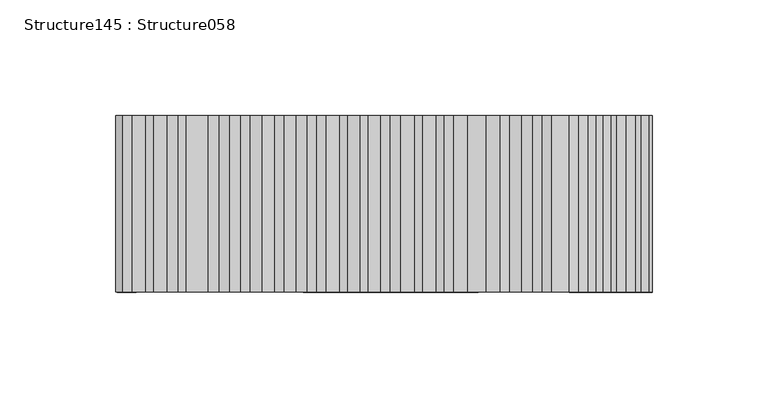
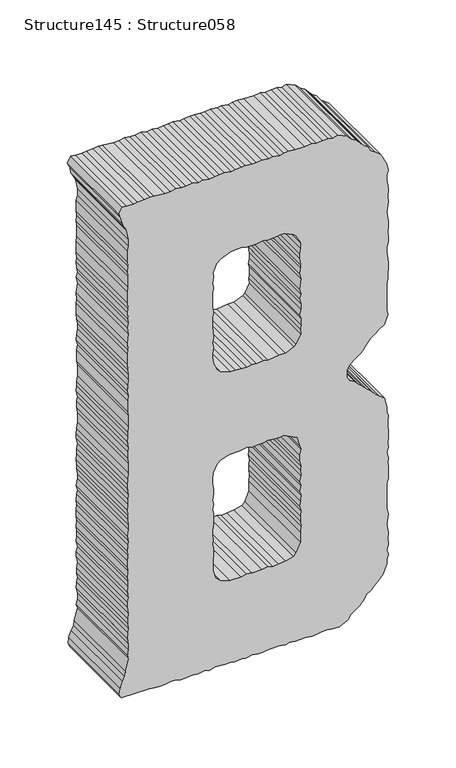
"""IFC4 building model written with IfcOpenShell, lengths in millimetres: proxy geometry, Structure145 : Structure058."""

from ifc_helpers import new_model, si_unit, frame, origin, place, context, project, spatial, polyline, outline, extrude, source, transform, mapped, element, save


def structure145_structure058_15f4931a(model_context):
    return source(origin(), model_context, "Body", "SweptSolid", [
        extrude(outline(polyline([(3581.5276686, -40098.3513957), (3585.0706354, -40095.4101556), (3593.2541183, -40091.9105132), (3597.3538828, -40091.9105132), (3601.4536473, -40090.7295243), (3606.1551384, -40091.9105132), (3610.838979, -40090.7295243), (3616.69739, -40091.331251), (3621.3732075, -40090.7295243), (3628.998288, -40091.9105132), (3638.3563415, -40090.7295243), (3644.2420307, -40091.9105132), (3666.5027089, -40091.9105132), (3670.5848228, -40090.7295243), (3681.1447249, -40090.7295243), (3684.6443673, -40091.331251), (3689.3458585, -40090.7295243), (3694.6298211, -40091.9105132), (3698.711935, -40090.7295243), (3703.4134261, -40091.331251), (3708.087639, -40090.7295243), (3713.3555556, -40090.7295243), (3718.0554422, -40091.331251), (3722.7312597, -40091.331251), (3727.4311462, -40090.7295243), (3730.9323932, -40091.9105132), (3735.6146291, -40091.9105132), (3744.4158848, -40094.2516312), (3747.9428055, -40098.3513957), (3750.3015741, -40101.8735025), (3754.9854146, -40105.3715403), (3757.3185096, -40108.9161117), (3761.418274, -40112.4141495), (3764.3611187, -40115.9362563), (3768.4432325, -40120.0360208), (3770.8036057, -40123.5581277), (3774.3032481, -40126.4769033), (3780.7441306, -40126.4769033), (3785.4456218, -40123.5581277), (3788.9452642, -40118.8550319), (3791.8865042, -40115.3569941), (3794.2292268, -40112.4141495), (3798.3305959, -40109.4953739), (3802.448011, -40105.973267), (3805.3459267, -40102.4527648), (3808.290376, -40098.9306579), (3811.2043377, -40094.2516312), (3819.4150989, -40091.331251), (3823.5341187, -40091.9105132), (3847.5598618, -40091.9105132), (3851.6612309, -40091.331251), (3856.9179152, -40091.331251), (3861.0192843, -40090.7295243), (3865.7015202, -40090.7295243), (3870.4030114, -40091.331251), (3875.686974, -40091.9105132), (3880.3627915, -40091.9105132), (3885.6210804, -40090.7295243), (3889.7208449, -40090.7295243), (3893.822214, -40091.331251), (3899.1061766, -40090.7295243), (3903.2059411, -40090.7295243), (3912.5896682, -40091.9105132), (3917.8479571, -40091.331251), (3921.9733953, -40090.7295243), (3926.6492128, -40091.331251), (3932.4899731, -40090.7295243), (3937.1930689, -40091.331251), (3940.718385, -40091.9105132), (3945.9766739, -40091.9105132), (3950.0940891, -40090.7295243), (3955.9348494, -40091.9105132), (3962.9774586, -40095.4101556), (3967.0788276, -40097.7721334), (3969.994394, -40101.8735025), (3972.9372387, -40105.973267), (3977.6194746, -40108.314385), (3979.3781211, -40111.8348872), (3982.8793681, -40114.7552674), (3987.0048063, -40118.2757697), (3989.3475288, -40122.3771388), (3993.4472933, -40126.4769033), (3996.9645864, -40134.0987746), (3995.7803883, -40138.2001437), (3996.390138, -40142.2999082), (3996.390138, -40147.003004), (3995.7803883, -40152.2628975), (3996.9645864, -40156.362662), (3996.390138, -40162.2242822), (3996.390138, -40170.4029513), (3996.9645864, -40176.287036), (3996.9645864, -40180.3868005), (3995.7803883, -40183.9089074), (3996.9645864, -40189.7705276), (3996.390138, -40193.2685654), (3996.9645864, -40199.1301856), (3996.390138, -40203.8108169), (3996.390138, -40207.9105814), (3996.9645864, -40213.1929394), (3996.9645864, -40216.7134417), (3996.390138, -40221.9957997), (3995.7803883, -40225.4938375), (3996.9645864, -40231.3554577), (3996.390138, -40235.4568268), (3996.390138, -40239.5565913), (3995.7803883, -40244.2596871), (3996.390138, -40249.5195806), (3995.7803883, -40253.6193451), (3996.9645864, -40258.9017031), (3996.390138, -40264.1615966), (3996.390138, -40268.2613611), (3996.9645864, -40272.9644569), (3995.7803883, -40277.6434836), (3995.7803883, -40282.3465794), (3996.9645864, -40291.7062374), (3996.9645864, -40295.2283443), (3996.390138, -40299.907371), (3996.390138, -40305.7689912), (3995.7803883, -40309.2910981), (3995.7803883, -40315.1511137), (3996.390138, -40319.2524828), (3991.0788971, -40322.1712584), (3986.4046842, -40319.831745), (3981.7208437, -40319.2524828), (3977.0209571, -40316.9129694), (3973.5197101, -40315.1511137), (3964.7361051, -40313.3683981), (3958.8776941, -40313.3683981), (3954.7506513, -40314.549387), (3944.8165449, -40314.549387), (3941.2912288, -40313.9701248), (3936.0345445, -40314.549387), (3931.9058971, -40313.9701248), (3921.9733953, -40313.9701248), (3917.8479571, -40314.549387), (3907.888177, -40314.549387), (3902.6314927, -40313.9701248), (3899.1061766, -40314.549387), (3893.246161, -40313.9701248), (3889.1463965, -40313.3683981), (3885.0626781, -40314.549387), (3879.1769888, -40313.3683981), (3870.9790644, -40314.549387), (3865.1190488, -40313.9701248), (3861.6178018, -40314.549387), (3852.2340747, -40314.549387), (3846.9757858, -40313.9701248), (3842.8583706, -40313.3683981), (3838.1761347, -40313.3683981), (3832.8921721, -40313.9701248), (3828.2163546, -40314.549387), (3823.5341187, -40313.3683981), (3818.8310229, -40313.9701248), (3808.8888934, -40313.9701248), (3805.3459267, -40313.3683981), (3795.4037973, -40313.3683981), (3790.1294623, -40313.9701248), (3786.6298199, -40313.9701248), (3781.9299333, -40314.549387), (3776.6427615, -40313.3683981), (3772.5606477, -40313.9701248), (3766.684586, -40313.9701248), (3762.0023501, -40313.3683981), (3753.2171405, -40313.3683981), (3747.9428055, -40313.9701248), (3743.2332913, -40314.549387), (3739.1592005, -40314.549387), (3733.8736333, -40313.3683981), (3729.7738688, -40313.9701248), (3725.0996559, -40313.9701248), (3719.8140887, -40314.549387), (3715.1302482, -40313.9701248), (3711.6145597, -40313.9701248), (3706.3289925, -40313.3683981), (3702.229228, -40313.3683981), (3696.3884676, -40314.549387), (3691.6869765, -40313.3683981), (3688.1873341, -40313.9701248), (3682.8857208, -40314.549387), (3678.81163, -40313.9701248), (3674.1277895, -40314.549387), (3668.2437048, -40314.549387), (3664.7440624, -40313.9701248), (3658.8840468, -40314.549387), (3655.3587307, -40313.9701248), (3650.6845178, -40313.9701248), (3645.4262289, -40314.549387), (3640.7167147, -40313.3683981), (3636.6153456, -40314.549387), (3631.915459, -40314.549387), (3626.0554434, -40313.3683981), (3621.3732075, -40313.9701248), (3616.69739, -40313.9701248), (3612.5976255, -40313.3683981), (3608.4705827, -40313.9701248), (3603.2122938, -40314.549387), (3598.5284533, -40313.3683981), (3593.2541183, -40313.3683981), (3588.5702778, -40314.549387), (3585.0706354, -40313.3683981), (3574.5107332, -40316.3112427), (3570.4109687, -40316.9129694), (3566.3095996, -40318.6732206), (3561.025637, -40320.9902694), (3555.7416744, -40321.5919961), (3551.6675836, -40319.831745), (3551.6675836, -40295.8076065), (3551.0658569, -40291.7062374), (3550.4833855, -40286.425484), (3551.0658569, -40282.3465794), (3551.6675836, -40277.0642214), (3551.6675836, -40272.9644569), (3550.4833855, -40268.8406233), (3550.4833855, -40264.1615966), (3551.0658569, -40259.4809653), (3550.4833855, -40254.1986073), (3551.6675836, -40248.9403184), (3550.4833855, -40244.2596871), (3551.6675836, -40239.5565913), (3551.6675836, -40236.0585535), (3551.0658569, -40230.753731), (3551.0658569, -40226.0747043), (3550.4833855, -40222.5525974), (3551.0658569, -40216.7134417), (3550.4833855, -40213.1929394), (3551.6675836, -40207.9105814), (3550.4833855, -40202.6506879), (3550.4833855, -40198.5509234), (3551.6675836, -40193.2685654), (3551.6675836, -40184.4881696), (3550.4833855, -40179.2058116), (3551.6675836, -40175.7077738), (3551.0658569, -40171.004678), (3551.0658569, -40161.64502), (3550.4833855, -40156.362662), (3551.0658569, -40151.6820307), (3551.6675836, -40148.139064), (3551.6675836, -40143.4584326), (3551.0658569, -40138.7794059), (3550.4833855, -40132.9177857), (3554.5831499, -40125.2959144), (3558.684519, -40122.9788655), (3561.025637, -40118.8550319), (3563.9412034, -40115.3569941), (3568.6426945, -40111.2331606), (3572.1423369, -40109.4953739), (3574.5107332, -40105.3715403), (3578.0103756, -40102.4527648), (3581.5276686, -40098.3513957)]), holes=[polyline([(3831.732043, -40166.3240467), (3827.6162325, -40165.72232), (3820.015221, -40169.8461536), (3818.2309008, -40171.5839402), (3815.3313805, -40179.2058116), (3815.3313805, -40184.4881696), (3814.148787, -40193.8478276), (3814.7296538, -40197.9716612), (3814.148787, -40203.8108169), (3814.7296538, -40207.9105814), (3814.148787, -40212.034415), (3814.148787, -40216.7134417), (3814.7296538, -40221.9957997), (3814.7296538, -40226.0747043), (3817.090027, -40234.2983024), (3820.5896694, -40237.2170779), (3827.0321565, -40240.1358535), (3832.8921721, -40241.318447), (3836.4174882, -40241.318447), (3841.6741725, -40240.1358535), (3845.8012153, -40241.318447), (3851.0595042, -40240.1358535), (3860.4432313, -40241.318447), (3869.2444869, -40241.318447), (3873.3185778, -40240.1358535), (3878.0024183, -40241.318447), (3892.0876365, -40241.318447), (3895.5888836, -40240.1358535), (3900.2887701, -40241.318447), (3904.9645876, -40240.1358535), (3909.6468235, -40240.7375802), (3916.6653636, -40237.7963402), (3919.6066036, -40234.2983024), (3923.1319197, -40226.0747043), (3923.7079727, -40221.394073), (3923.7079727, -40216.7134417), (3922.5494483, -40213.1929394), (3922.5494483, -40203.8108169), (3923.7079727, -40197.9716612), (3922.5494483, -40193.8478276), (3923.1319197, -40188.5879341), (3923.7079727, -40183.9089074), (3923.7079727, -40179.7850738), (3920.2067257, -40172.1856669), (3917.8479571, -40169.8461536), (3910.8310217, -40166.3240467), (3905.5470591, -40166.3240467), (3900.8648231, -40166.9049135), (3896.763454, -40166.9049135), (3890.905043, -40166.3240467), (3887.9621984, -40166.3240467), (3882.7039095, -40166.9049135), (3878.0024183, -40165.72232), (3868.6443649, -40166.9049135), (3863.9332461, -40165.72232), (3860.4432313, -40166.9049135), (3855.1769193, -40165.72232), (3850.4754282, -40165.72232), (3845.1914656, -40166.9049135), (3842.2758992, -40165.72232), (3836.4174882, -40165.72232), (3831.732043, -40166.3240467)]), polyline([(3736.7988273, -40172.7649292), (3735.0578314, -40169.2668914), (3726.8566978, -40166.9049135), (3723.3313817, -40165.72232), (3718.6571688, -40166.9049135), (3712.7971532, -40166.9049135), (3708.087639, -40165.72232), (3704.5879966, -40166.3240467), (3699.3136616, -40165.72232), (3694.6298211, -40166.9049135), (3690.512406, -40165.72232), (3685.2444894, -40166.9049135), (3681.7271964, -40165.72232), (3676.4432338, -40166.3240467), (3672.3691429, -40166.9049135), (3667.6853024, -40165.72232), (3662.9854159, -40166.3240467), (3658.3015753, -40166.3240467), (3653.6000842, -40165.72232), (3648.3161216, -40166.3240467), (3639.5405396, -40166.3240467), (3631.3410106, -40169.8461536), (3628.4158166, -40172.1856669), (3626.6571701, -40179.2058116), (3626.0554434, -40185.0674318), (3625.472972, -40189.7705276), (3626.6571701, -40193.8478276), (3626.0554434, -40199.1301856), (3626.0554434, -40207.9105814), (3626.6571701, -40212.6136772), (3625.472972, -40217.2927039), (3625.472972, -40226.676431), (3628.4158166, -40234.8775646), (3631.915459, -40238.3756024), (3639.5405396, -40240.7375802), (3648.9258713, -40240.7375802), (3654.1841602, -40240.1358535), (3658.8840468, -40240.1358535), (3663.5598643, -40241.318447), (3667.6853024, -40240.7375802), (3671.7690209, -40241.318447), (3676.4432338, -40241.318447), (3681.7271964, -40240.1358535), (3690.512406, -40240.1358535), (3695.2122926, -40241.318447), (3699.3136616, -40240.1358535), (3703.4134261, -40241.318447), (3709.2718371, -40240.1358535), (3713.3555556, -40240.1358535), (3718.0554422, -40241.318447), (3723.3313817, -40241.318447), (3728.0152223, -40240.7375802), (3735.0578314, -40237.2170779), (3737.400554, -40234.2983024), (3739.7416719, -40226.676431), (3739.7416719, -40217.8719661), (3740.9162424, -40212.034415), (3739.7416719, -40207.9105814), (3740.3161203, -40203.2299501), (3740.3161203, -40197.9716612), (3740.9162424, -40193.8478276), (3740.3161203, -40188.5879341), (3740.3161203, -40183.9089074), (3740.9162424, -40180.3868005), (3736.7988273, -40172.7649292)])]), frame((0.0, 247945.1599557, 0.0), z_axis=(0.0, 1.0, 0.0), x_axis=(0.0, 0.0, 1.0)), (0.0, 0.0, 1.0), 76.2),
    ])


if __name__ == "__main__":
    model = new_model("IFC4")
    model_context = context("Model", 3, world=origin())
    ifc_project = project(units=[si_unit("LENGTHUNIT", "METRE", prefix="MILLI")], contexts=[model_context])
    site = spatial("IfcSite", under=ifc_project)
    building = spatial("IfcBuilding", under=site)
    placement = place(None, origin())
    structure145_structure058_shape = structure145_structure058_15f4931a(model_context)
    element("IfcBuildingElementProxy", 1, Name="Structure145 : Structure058", ObjectType="Structure145 : Structure058", at=placement, inside=building, context=model_context, shape_type="MappedRepresentation", body=[
        mapped(structure145_structure058_shape, transform((0.0, 0.0, 0.0), x_axis=(1.0, 0.0, 0.0), y_axis=(0.0, 1.0, 0.0), z_axis=(0.0, 0.0, 1.0))),
    ])
    save(model, "model.ifc")

# Revit data of these elements
# Type "Structure145 : Structure058"
#   NameOverride = "Structure058"
# Element 1 (IfcBuildingElementProxy, "Structure145 : Structure058")
#   Materials on its faces: "BRUSHED ALUM. LETTERING"
# Materials
#   "BRUSHED ALUM. LETTERING": class "Unassigned", colour RGB 169 181 186, transparency 0, Cost = 0
